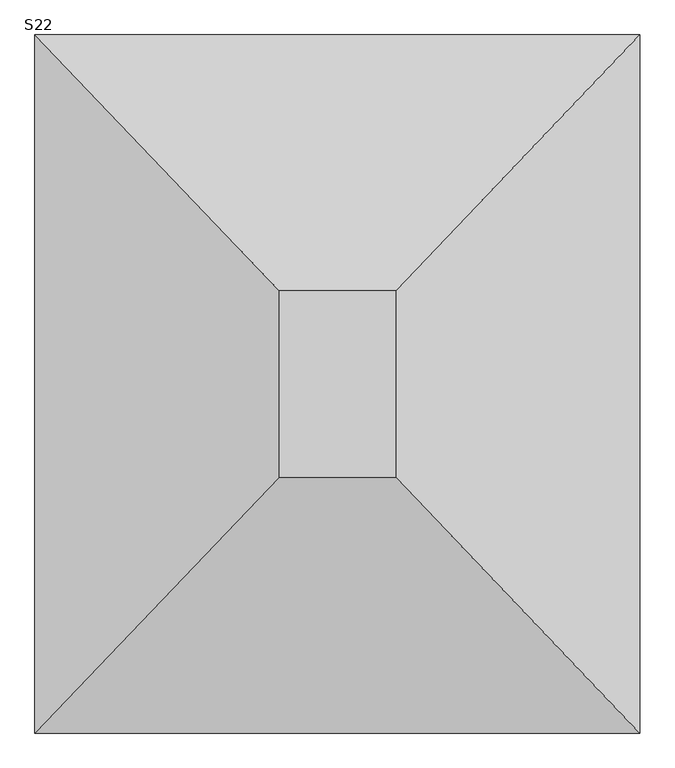
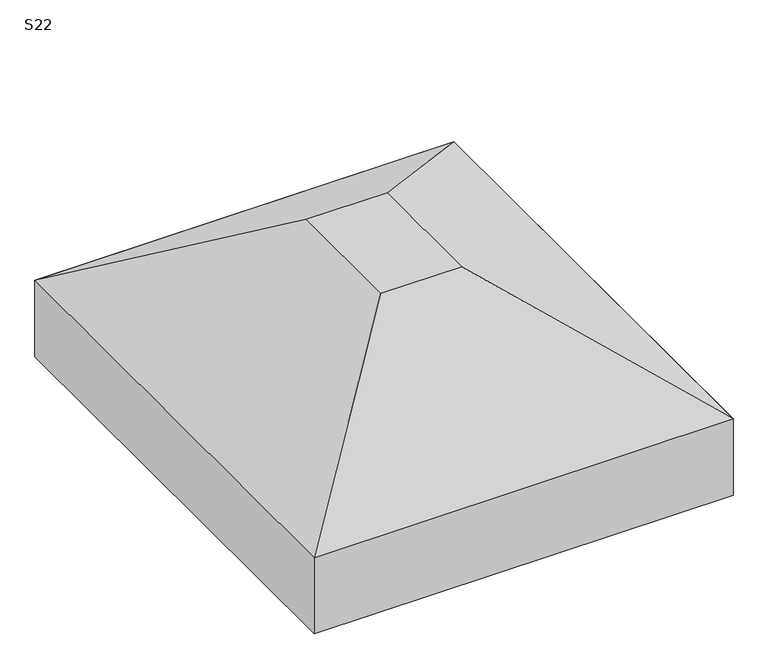
"""IFC4 building model written with IfcOpenShell, lengths in millimetres: fastener geometry, TQS - Sapata : S22."""

from ifc_helpers import new_model, si_unit, frame, origin, place, context, project, spatial, polyline, outline, extrude, faceted_brep, source, transform, mapped, element, save


def s22_9d23c3d3(model_context):
    return source(origin(), model_context, "Body", "SolidModel", [
        faceted_brep([(-75.0, 0.0, 0.0), (-325.0, 0.0, 0.0), (-325.0, -400.0, 0.0), (-75.0, -400.0, 0.0), (450.0, 550.0, -350.0), (450.0, -950.0, -350.0), (-850.0, -950.0, -350.0), (-850.0, 550.0, -350.0)], [[[0, 1, 2, 3]], [[4, 5, 6, 7]], [[4, 7, 1, 0]], [[7, 6, 2, 1]], [[6, 5, 3, 2]], [[5, 4, 0, 3]]]),
        extrude(outline(polyline([(450.0, 550.0), (450.0, -950.0), (-850.0, -950.0), (-850.0, 550.0), (450.0, 550.0)])), frame((0.0, 0.0, -600.0), z_axis=(0.0, 0.0, 1.0), x_axis=(1.0, 0.0, 0.0)), (0.0, 0.0, 1.0), 250.0),
    ])


if __name__ == "__main__":
    model = new_model("IFC4")
    model_context = context("Model", 3, world=origin())
    ifc_project = project(units=[si_unit("LENGTHUNIT", "METRE", prefix="MILLI")], contexts=[model_context])
    site = spatial("IfcSite", under=ifc_project)
    building = spatial("IfcBuilding", under=site)
    placement = place(None, origin())
    s22_shape = s22_9d23c3d3(model_context)
    element("IfcFastener", 1, ObjectType="TQS - Sapata : S22", at=placement, inside=building, context=model_context, shape_type="MappedRepresentation", body=[
        mapped(s22_shape, transform((0.0, 0.0, 0.0), x_axis=(1.0, 0.0, 0.0), y_axis=(0.0, 1.0, 0.0), z_axis=(0.0, 0.0, 1.0))),
    ])
    save(model, "model.ifc")

# Revit data of these elements
# Type "TQS - Sapata : S22"
#   TY = 0.40 m
#   TX = 0.25 m
#   HS = 0.60 m
#   H0 = 0.25 m
#   EXCYABS = 0.75 m
#   EXCY = 0.00 m
#   EXCXABS = 0.65 m
#   EXCX = 0.00 m
#   DIMY = 1.50 m
#   DIMX = 1.30 m
#   Material estrutural = Concreto - Concreto concretado no local
#   Width = 0
#   Length = 0
# Element 1 (IfcFastener, "TQS - Sapata : S22")
#   Materials on its faces: "Concreto - Concreto concretado no local"
# Materials
#   "Concreto - Concreto concretado no local": class "Concreto", colour RGB 192 192 192, transparency 0
